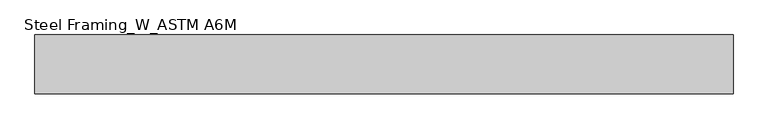
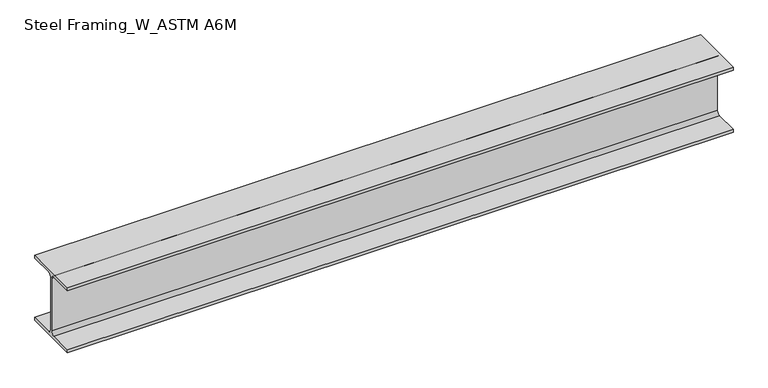
"""IFC4 building model written with IfcOpenShell, lengths in millimetres: beam geometry, Steel Framing_W_ASTM A6M : H_SB_AR_S02_W250x49.1_RCG1."""

from ifc_helpers import new_model, si_unit, point, frame, frame_2d, origin, place, context, project, spatial, polyline, circle_curve, trimmed, segment, composite_curve, outline, extrude, source, transform, mapped, element, save


def steel_framing_w_astm_a6m_c3bcebff(model_context):
    return source(origin(), model_context, "Body", "SweptSolid", [
        extrude(outline(composite_curve([segment(polyline([(101.0, -112.5), (101.0, -123.5), (-101.0, -123.5), (-101.0, -112.5), (-16.385, -112.5)]), True, "CONTINUOUS"), segment(trimmed(circle_curve(frame_2d((-16.385, -99.8)), 12.7), [point((-16.385, -112.5))], [point((-3.685, -99.8))], True, "CARTESIAN"), True, "CONTINUOUS"), segment(polyline([(-3.685, -99.8), (-3.685, 99.8)]), True, "CONTINUOUS"), segment(trimmed(circle_curve(frame_2d((-16.385, 99.8)), 12.7), [point((-3.685, 99.8))], [point((-16.385, 112.5))], True, "CARTESIAN"), True, "CONTINUOUS"), segment(polyline([(-16.385, 112.5), (-101.0, 112.5), (-101.0, 123.5), (101.0, 123.5), (101.0, 112.5), (16.385, 112.5)]), True, "CONTINUOUS"), segment(trimmed(circle_curve(frame_2d((16.385, 99.8)), 12.7), [point((16.385, 112.5))], [point((3.685, 99.8))], True, "CARTESIAN"), True, "CONTINUOUS"), segment(polyline([(3.685, 99.8), (3.685, -99.8)]), True, "CONTINUOUS"), segment(trimmed(circle_curve(frame_2d((16.385, -99.8)), 12.7), [point((3.685, -99.8))], [point((16.385, -112.5))], True, "CARTESIAN"), True, "CONTINUOUS"), segment(polyline([(16.385, -112.5), (101.0, -112.5)]), True, "CONTINUOUS")], self_intersect=False)), frame((-1243.5, 0.0, 0.0), z_axis=(1.0, 0.0, 0.0), x_axis=(0.0, 1.0, 0.0)), (0.0, 0.0, 1.0), 2391.9525253),
    ])


if __name__ == "__main__":
    model = new_model("IFC4")
    model_context = context("Model", 3, world=origin())
    ifc_project = project(units=[si_unit("LENGTHUNIT", "METRE", prefix="MILLI")], contexts=[model_context])
    site = spatial("IfcSite", under=ifc_project)
    building = spatial("IfcBuilding", under=site)
    placement = place(None, origin())
    steel_framing_w_astm_a6m_shape = steel_framing_w_astm_a6m_c3bcebff(model_context)
    element("IfcBeam", 1, ObjectType="Steel Framing_W_ASTM A6M : H_SB_AR_S02_W250x49.1_RCG1", at=placement, inside=building, context=model_context, shape_type="MappedRepresentation", body=[
        mapped(steel_framing_w_astm_a6m_shape, transform((0.0, 0.0, 0.0), x_axis=(1.0, 0.0, 0.0), y_axis=(0.0, 1.0, 0.0), z_axis=(0.0, 0.0, 1.0))),
    ])
    save(model, "model.ifc")

# Revit data of these elements
# Type "Steel Framing_W_ASTM A6M : H_SB_AR_S02_W250x49.1_RCG1"
#   Section Name Key = "W10x33"
#   Width = 20.2 cm
#   Web Thickness = 0.737 cm
#   Web Fillet = 1.27 cm
#   Warping Constant = 212000.0 cm⁶
#   Torsional Moment of Inertia = 24.30 cm⁴
#   Section Area = 62.6 cm²
#   Plastic Modulus weak axis = 229.0 cm³
#   Plastic Modulus strong axis = 636.0 cm³
#   Perimeter = 1.27 m²/m
#   Nominal Weight = 49.10 kgf/m
#   Moment of Inertia weak axis = 1520.00 cm⁴
#   Moment of Inertia strong axis = 7120.00 cm⁴
#   Height = 24.7 cm
#   Flange Thickness = 1.1 cm
#   Elastic Modulus weak axis = 151.0 cm³
#   Elastic Modulus strong axis = 574.0 cm³
#   Centroid Vertical = 12.35 cm
#   Centroid Horizontal = 10.1 cm
#   Length [instance default] = 1500 mm
#   Structural Material [instance default] = Steel, 45-345
#   Bolt Spacing = 0
#   Assembly Code = ""
# Element 1 (IfcBeam, "Steel Framing_W_ASTM A6M : H_SB_AR_S02_W250x49.1_RCG1")
#   Materials on its faces: "Steel, 45-345"
# Materials
#   "Steel, 45-345": class "Metal", colour RGB 189 187 185, transparency 0, Description = "Steel 345 MPa", Cost = 0
